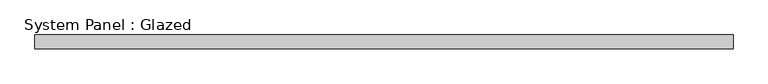
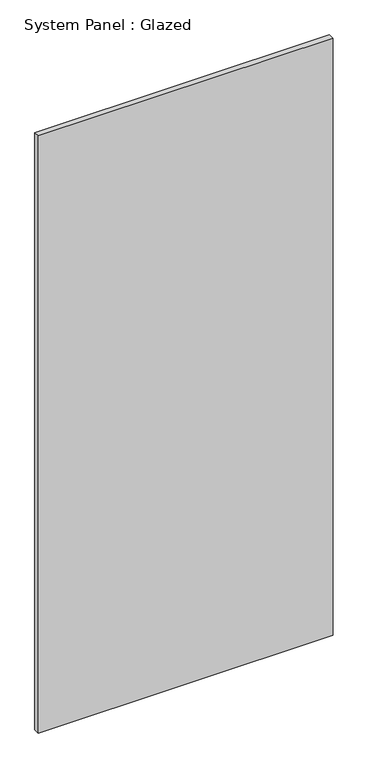
"""IFC4 building model written with IfcOpenShell, lengths in millimetres: plate geometry, System Panel : Glazed."""

from ifc_helpers import new_model, si_unit, origin, origin_with_axes, place, context, project, spatial, polyline, outline, extrude, source, transform, mapped, element, save


def system_panel_glazed_3a20483a(model_context):
    return source(origin(), model_context, "Body", "SweptSolid", [
        extrude(outline(polyline([(651.3841868, 19.05), (-651.3841868, 19.05), (-651.3841868, 44.45), (651.3841868, 44.45), (651.3841868, 19.05)])), origin_with_axes(), (0.0, 0.0, 1.0), 2788.92),
    ])


if __name__ == "__main__":
    model = new_model("IFC4")
    model_context = context("Model", 3, world=origin())
    ifc_project = project(units=[si_unit("LENGTHUNIT", "METRE", prefix="MILLI")], contexts=[model_context])
    site = spatial("IfcSite", under=ifc_project)
    building = spatial("IfcBuilding", under=site)
    placement = place(None, origin())
    system_panel_glazed_shape = system_panel_glazed_3a20483a(model_context)
    element("IfcPlate", 1, ObjectType="System Panel : Glazed", at=placement, inside=building, context=model_context, shape_type="MappedRepresentation", body=[
        mapped(system_panel_glazed_shape, transform((0.0, 0.0, 0.0), x_axis=(1.0, 0.0, 0.0), y_axis=(0.0, 1.0, 0.0), z_axis=(0.0, 0.0, 1.0))),
    ])
    save(model, "model.ifc")

# Revit data of these elements
# Type "System Panel : Glazed"
#   Construction Type Id = "GSP4R"
#   Analytic Construction = "1/8 in Pilkington single glazing"
#   Visual Light Transmittance = 0.9
#   Solar Heat Gain Coefficient = 0.86
#   Heat Transfer Coefficient (U) = 1.18115 BTU/(h·ft²·°F)
#   Define Thermal Properties by = 1
# Element 1 (IfcPlate, "System Panel : Glazed")
#   Materials on its faces: "Glass"
# Materials
#   "Glass": class "Glass", colour RGB 0 128 192, transparency 0.75, Description = "Soda Lime Glass", Cost = 0
